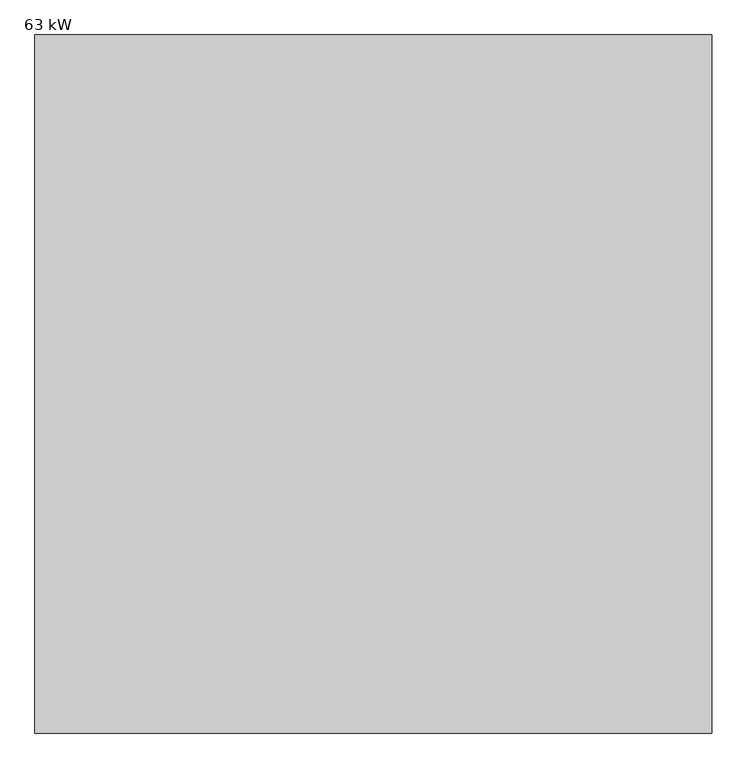
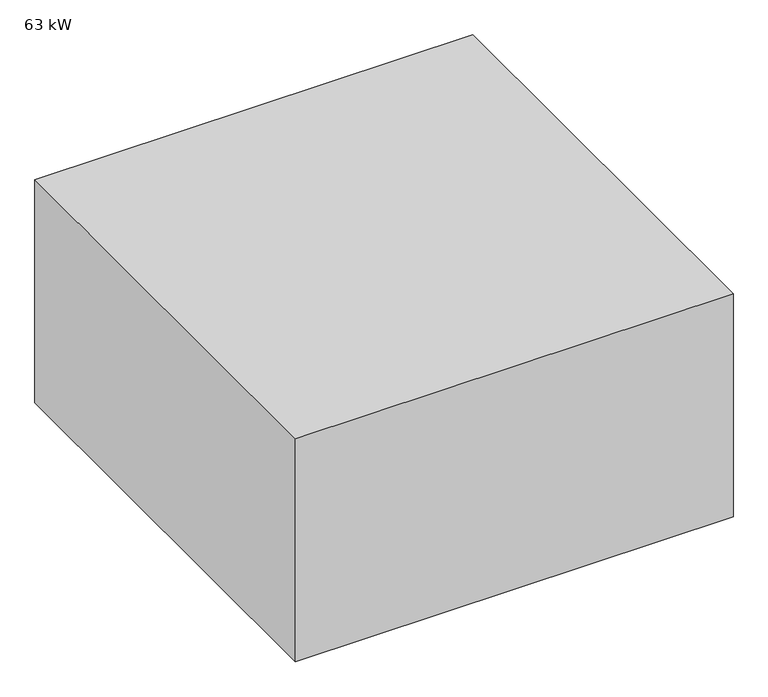
"""IFC4 building model written with IfcOpenShell, lengths in millimetres: proxy geometry, M_Rooftop AC Unit - 53-88 kW - Bottom Return Connection : 63 kW."""

from ifc_helpers import new_model, si_unit, origin, place, context, project, spatial, faceted_brep, source, transform, mapped, element, save


def proxy_63_kw_72c3e3c2(model_context):
    return source(origin(), model_context, "Body", "Brep", [
        faceted_brep([(-2120.9, 0.0, 1143.0), (0.0, 0.0, 1143.0), (0.0, 2187.6, 1143.0), (-2120.9, 2187.6, 1143.0), (-2120.9, 0.0, 0.0), (-2120.9, 2187.6, 0.0), (0.0, 2187.6, 0.0), (0.0, 0.0, 0.0), (-1443.0, 274.6, 0.0), (-935.0, 274.6, 0.0), (-935.0, 2001.8, 0.0), (-1443.0, 2001.8, 0.0), (-100.0, 2036.8, 0.0), (-531.8, 2036.8, 0.0), (-531.8, 284.2, 0.0), (-100.0, 284.2, 0.0), (-1443.0, 274.6, 25.4), (-1443.0, 2001.8, 25.4), (-935.0, 2001.8, 25.4), (-935.0, 274.6, 25.4), (-100.0, 2036.8, 25.4), (-100.0, 284.2, 25.4), (-531.8, 284.2, 25.4), (-531.8, 2036.8, 25.4)], [[[0, 1, 2, 3]], [[4, 5, 6, 7], [8, 9, 10, 11], [12, 13, 14, 15]], [[1, 0, 4, 7]], [[2, 1, 7, 6]], [[3, 2, 6, 5]], [[0, 3, 5, 4]], [[16, 17, 18, 19]], [[16, 19, 9, 8]], [[19, 18, 10, 9]], [[18, 17, 11, 10]], [[17, 16, 8, 11]], [[20, 21, 22, 23]], [[20, 23, 13, 12]], [[23, 22, 14, 13]], [[22, 21, 15, 14]], [[21, 20, 12, 15]]]),
    ])


if __name__ == "__main__":
    model = new_model("IFC4")
    model_context = context("Model", 3, world=origin())
    ifc_project = project(units=[si_unit("LENGTHUNIT", "METRE", prefix="MILLI")], contexts=[model_context])
    site = spatial("IfcSite", under=ifc_project)
    building = spatial("IfcBuilding", under=site)
    placement = place(None, origin())
    proxy_63_kw_shape = proxy_63_kw_72c3e3c2(model_context)
    element("IfcBuildingElementProxy", 1, Name="M_Rooftop AC Unit - 53-88 kW - Bottom Return Connection : 63 kW", ObjectType="M_Rooftop AC Unit - 53-88 kW - Bottom Return Connection : 63 kW", at=placement, inside=building, context=model_context, shape_type="MappedRepresentation", body=[
        mapped(proxy_63_kw_shape, transform((0.0, 0.0, 0.0), x_axis=(1.0, 0.0, 0.0), y_axis=(0.0, 1.0, 0.0), z_axis=(0.0, 0.0, 1.0))),
    ])
    save(model, "model.ifc")

# Revit data of these elements
# Project information
#   Project Issue Date = "Issue Date"
#   Project Status = "Project Status"
#   Client Name = "Owner"
#   Project Address = "Enter address here"
#   Project Name = "Project Name"
#   Project Number = "Project Number"
# Type "M_Rooftop AC Unit - 53-88 kW - Bottom Return Connection : 63 kW"
#   PartShape = "Rectangular Duct"
#   Voltage [instance default] = 460 V
#   SupplyX = 508 mm
#   UnitWidth = 2120.9 mm
#   UnitHeight = 1143 mm
#   UnitDepth = 2187.6 mm
#   SupplyYOffset = 274.6 mm
#   SupplyXOffset = 935 mm
#   ReturnYOffset = 150.8 mm
#   ReturnXOffset = 100 mm
#   Min Flow = 5400
#   Max Flow = 9000
#   SupplyY = 1727.2 mm
#   ReturnX = 431.8 mm
#   ReturnY = 1752.6 mm
#   External Static Pressure [instance default] = 99.54 Pa
#   Apparent Load [instance default] = 20000 VA
#   AirFlow - Supply [instance default] = 3398.02 L/s
#   AirFlow - Return [instance default] = 3398.02 L/s
#   Supply/Return Symbols [instance default] = yes
#   Number of Poles [instance default] = 3
#   Load Classification = Cooling
#   Model = ""
#   Default Elevation = 0
#   Assembly Code = ""
